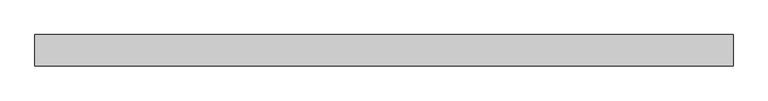
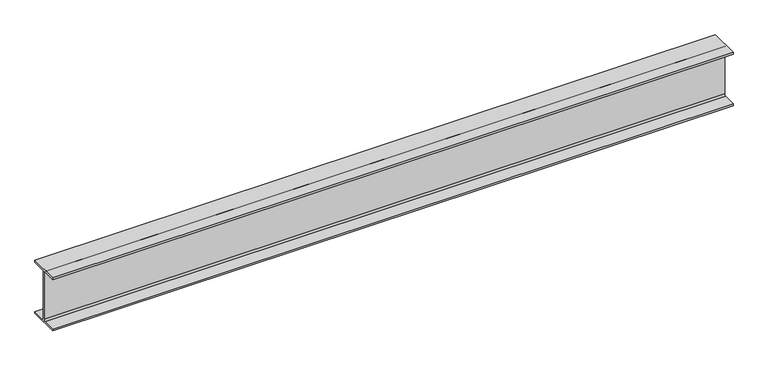
"""IFC4 building model written with IfcOpenShell, lengths in millimetres: beam geometry, Old_Steel Beam_H-KSD3502 : H_SB_ASB_H-200×200x8x12."""

import ifcopenshell
import ifcopenshell.guid

model = None  # the IFC model being written
_history = None  # IfcOwnerHistory: only IFC2X3 demands one
_inside = {}  # id of a spatial element -> (the spatial element, [elements in it])
_under = {}  # id of a project, library or spatial element -> (it, [spatial elements below it])
_declared = {}  # id of a project -> (the project, [libraries it declares])
_typed = {}  # id of a type object -> (the type object, [elements of that type])
_made_of = {}  # id of a material, layer set ... -> (it, [elements and type objects made of it])


def new_model(schema):
    """Start an empty IFC model of exactly this schema.

    Asked for "IFC4X3", IfcOpenShell would pick the latest addendum, in which some entities
    have other attributes; the version numbers below select the first issue.
    IFC2X3 requires an IfcOwnerHistory on every rooted entity: one is made here for all.
    """
    global model, _history
    if schema == "IFC4X3":
        model = ifcopenshell.file(schema_version=(4, 3, 0, 0))
    else:
        model = ifcopenshell.file(schema=schema)
    _inside.clear()
    _under.clear()
    _declared.clear()
    _typed.clear()
    _made_of.clear()
    _history = None
    if model.schema == "IFC2X3":
        org = make("IfcOrganization", Name="unknown")
        user = make(
            "IfcPersonAndOrganization",
            ThePerson=make("IfcPerson", FamilyName="unknown"),
            TheOrganization=org,
        )
        app = make(
            "IfcApplication",
            ApplicationDeveloper=org,
            Version="unknown",
            ApplicationFullName="unknown",
            ApplicationIdentifier="unknown",
        )
        _history = make(
            "IfcOwnerHistory",
            OwningUser=user,
            OwningApplication=app,
            ChangeAction="ADDED",
            CreationDate=0,
        )
    return model


def make(cls, **values):
    """One entity of the class cls with the attributes given. An attribute that is None is left unset."""
    return model.create_entity(
        cls, **{name: value for name, value in values.items() if value is not None}
    )


def rooted(cls, **values):
    """An entity with a GlobalId (a new one), such as an element, a storey or a relation."""
    return make(cls, GlobalId=ifcopenshell.guid.new(), OwnerHistory=_history, **values)


def si_unit(unit_type, name, prefix=None):
    """IfcSIUnit, for example si_unit("LENGTHUNIT", "METRE", prefix="MILLI")."""
    return make("IfcSIUnit", UnitType=unit_type, Prefix=prefix, Name=name)


def assignment(units):
    """IfcUnitAssignment: the units of a project."""
    return None if units is None else make("IfcUnitAssignment", Units=units)


def point(xyz):
    """IfcCartesianPoint."""
    return None if xyz is None else make("IfcCartesianPoint", Coordinates=xyz)


def direction(xyz):
    """IfcDirection."""
    return None if xyz is None else make("IfcDirection", DirectionRatios=xyz)


def frame(location, z_axis=None, x_axis=None):
    """IfcAxis2Placement3D, a coordinate frame: its origin and axes. An axis left out is left unset."""
    return make(
        "IfcAxis2Placement3D",
        Location=point(location),
        Axis=direction(z_axis),
        RefDirection=direction(x_axis),
    )


def frame_2d(location, x_axis=None):
    """IfcAxis2Placement2D, a coordinate frame in the plane: its origin and x axis."""
    return make(
        "IfcAxis2Placement2D", Location=point(location), RefDirection=direction(x_axis)
    )


def origin():
    """The frame at (0, 0, 0) with its axes left unset."""
    return frame((0.0, 0.0, 0.0))


def place(relative_to, where):
    """IfcLocalPlacement: puts the frame where relative to a parent placement (None: the world)."""
    return make(
        "IfcLocalPlacement", PlacementRelTo=relative_to, RelativePlacement=where
    )


def context(
    kind, dimensions, precision=None, world=None, true_north=None, identifier=None
):
    """IfcGeometricRepresentationContext, for example the 3D "Model" context."""
    return make(
        "IfcGeometricRepresentationContext",
        ContextIdentifier=identifier,
        ContextType=kind,
        CoordinateSpaceDimension=dimensions,
        Precision=precision,
        WorldCoordinateSystem=world,
        TrueNorth=true_north,
    )


def project(units=None, contexts=None):
    """IfcProject with its units and contexts."""
    return rooted(
        "IfcProject",
        Name="project",
        RepresentationContexts=contexts,
        UnitsInContext=assignment(units),
    )


def spatial(cls, under=None, at=None, **own):
    """A site, building, storey or space (cls), placed at a placement, below another one or the project."""
    s = rooted(cls, ObjectPlacement=at, **own)
    if under is not None:
        _under.setdefault(under.id(), (under, []))[1].append(s)
    return s


def polyline(points):
    """IfcPolyline through the points."""
    return make("IfcPolyline", Points=[point(p) for p in points])


def circle_curve(where, radius):
    """IfcCircle in the frame where."""
    return make("IfcCircle", Position=where, Radius=radius)


def trimmed(basis, trim1, trim2, sense, master):
    """IfcTrimmedCurve: the piece of a basis curve between two trims."""
    return make(
        "IfcTrimmedCurve",
        BasisCurve=basis,
        Trim1=trim1,
        Trim2=trim2,
        SenseAgreement=sense,
        MasterRepresentation=master,
    )


def segment(curve, same_sense, transition):
    """IfcCompositeCurveSegment."""
    return make(
        "IfcCompositeCurveSegment",
        Transition=transition,
        SameSense=same_sense,
        ParentCurve=curve,
    )


def composite_curve(segments, self_intersect=None):
    """IfcCompositeCurve: segments joined end to end."""
    return make("IfcCompositeCurve", Segments=segments, SelfIntersect=self_intersect)


def outline(outer, holes=None, kind="AREA"):
    """IfcArbitraryClosedProfileDef: a profile drawn as a closed curve; with holes, ...WithVoids."""
    if holes is None:
        return make("IfcArbitraryClosedProfileDef", ProfileType=kind, OuterCurve=outer)
    return make(
        "IfcArbitraryProfileDefWithVoids",
        ProfileType=kind,
        OuterCurve=outer,
        InnerCurves=holes,
    )


def extrude(swept, where, along, depth):
    """IfcExtrudedAreaSolid: the profile swept, set in the frame where, extruded along a direction by depth."""
    return make(
        "IfcExtrudedAreaSolid",
        SweptArea=swept,
        Position=where,
        ExtrudedDirection=direction(along),
        Depth=depth,
    )


def shape(context_of_items, identifier, shape_type, items):
    """IfcShapeRepresentation: the items that make up one representation, for example the "Body"."""
    return make(
        "IfcShapeRepresentation",
        ContextOfItems=context_of_items,
        RepresentationIdentifier=identifier,
        RepresentationType=shape_type,
        Items=items,
    )


def source(mapping_origin, context_of_items, identifier, shape_type, items):
    """IfcRepresentationMap: a shape defined once, which mapped items show again and again."""
    return make(
        "IfcRepresentationMap",
        MappingOrigin=mapping_origin,
        MappedRepresentation=shape(context_of_items, identifier, shape_type, items),
    )


def transform(
    local_origin,
    x_axis=None,
    y_axis=None,
    z_axis=None,
    scale=None,
    scale2=None,
    scale3=None,
    uniform=True,
):
    """IfcCartesianTransformationOperator3D, or its non-uniform kind. x_axis, y_axis, z_axis: its Axis1, 2, 3."""
    if uniform:
        return make(
            "IfcCartesianTransformationOperator3D",
            Axis1=direction(x_axis),
            Axis2=direction(y_axis),
            LocalOrigin=point(local_origin),
            Scale=scale,
            Axis3=direction(z_axis),
        )
    return make(
        "IfcCartesianTransformationOperator3DnonUniform",
        Axis1=direction(x_axis),
        Axis2=direction(y_axis),
        LocalOrigin=point(local_origin),
        Scale=scale,
        Axis3=direction(z_axis),
        Scale2=scale2,
        Scale3=scale3,
    )


def mapped(mapping_source, mapping_target):
    """IfcMappedItem: shows the shape of a source again, moved by a transform."""
    return make(
        "IfcMappedItem", MappingSource=mapping_source, MappingTarget=mapping_target
    )


def made_of(thing, what):
    """Note that an element or type object is made of a material, layer set ...; save() writes the relation."""
    if what is not None:
        _made_of.setdefault(what.id(), (what, []))[1].append(thing)
    return thing


def element(
    cls,
    number,
    at=None,
    inside=None,
    cuts=None,
    type_object=None,
    material=None,
    context=None,
    identifier="Body",
    shape_type=None,
    held_by="IfcProductDefinitionShape",
    body=None,
    shapes=None,
    **own,
):
    """One element of the class cls, such as IfcWall. Its Tag is "e" and its number.

    at: its placement. inside: the storey or other place that contains it. cuts: it is an
    opening in that element (IfcRelVoidsElement). A single representation is given by context,
    identifier, shape_type and body (its items); several are given by shapes. held_by: the class
    of the entity that holds the representations. save() writes the other relations.
    """
    e = rooted(cls, Tag="e%d" % number, ObjectPlacement=at, **own)
    if body is not None:
        shapes = [shape(context, identifier, shape_type, body)]
    if shapes is not None:
        e.Representation = make(held_by, Representations=shapes)
    if inside is not None:
        _inside.setdefault(inside.id(), (inside, []))[1].append(e)
    if cuts is not None:
        rooted(
            "IfcRelVoidsElement", RelatingBuildingElement=cuts, RelatedOpeningElement=e
        )
    if type_object is not None:
        _typed.setdefault(type_object.id(), (type_object, []))[1].append(e)
    return made_of(e, material)


def aggregate(whole, parts):
    """IfcRelAggregates: a whole, such as a stair, and the parts it consists of."""
    return rooted("IfcRelAggregates", RelatingObject=whole, RelatedObjects=parts)


def save(model, path):
    """Write the relations noted so far, then the file.

    IfcRelAggregates (storeys below a building ...), IfcRelContainedInSpatialStructure (elements
    in a storey), IfcRelDefinesByType, IfcRelAssociatesMaterial and IfcRelDeclares: one each for
    every whole, place, type object, material and project.
    """
    for whole, parts in _under.values():
        aggregate(whole, parts)
    for where, things in _inside.values():
        rooted(
            "IfcRelContainedInSpatialStructure",
            RelatedElements=things,
            RelatingStructure=where,
        )
    for kind, things in _typed.values():
        rooted("IfcRelDefinesByType", RelatedObjects=things, RelatingType=kind)
    for what, things in _made_of.values():
        rooted("IfcRelAssociatesMaterial", RelatedObjects=things, RelatingMaterial=what)
    for by, libraries in _declared.values():
        rooted("IfcRelDeclares", RelatingContext=by, RelatedDefinitions=libraries)
    model.write(path)


def beam_556eb451(model_context):
    return source(origin(), model_context, "Body", "SweptSolid", [
        extrude(outline(composite_curve([segment(polyline([(-82.5, -141.5), (-11.9, -141.5)]), True, "CONTINUOUS"), segment(trimmed(circle_curve(frame_2d((-11.9, -132.6)), 8.9), [point((-11.9, -141.5))], [point((-3.0, -132.6))], True, "CARTESIAN"), True, "CONTINUOUS"), segment(polyline([(-3.0, -132.6), (-3.0, 132.6)]), True, "CONTINUOUS"), segment(trimmed(circle_curve(frame_2d((-11.9, 132.6)), 8.9), [point((-3.0, 132.6))], [point((-11.9, 141.5))], True, "CARTESIAN"), True, "CONTINUOUS"), segment(polyline([(-11.9, 141.5), (-82.5, 141.5), (-82.5, 151.7), (82.5, 151.7), (82.5, 141.5), (11.9, 141.5)]), True, "CONTINUOUS"), segment(trimmed(circle_curve(frame_2d((11.9, 132.6)), 8.9), [point((11.9, 141.5))], [point((3.0, 132.6))], True, "CARTESIAN"), True, "CONTINUOUS"), segment(polyline([(3.0, 132.6), (3.0, -132.6)]), True, "CONTINUOUS"), segment(trimmed(circle_curve(frame_2d((11.9, -132.6)), 8.9), [point((3.0, -132.6))], [point((11.9, -141.5))], True, "CARTESIAN"), True, "CONTINUOUS"), segment(polyline([(11.9, -141.5), (82.5, -141.5), (82.5, -151.7), (-82.5, -151.7), (-82.5, -141.5)]), True, "CONTINUOUS")], self_intersect=False)), frame((-1848.779151, 0.0, 0.0), z_axis=(1.0, 0.0, 0.0), x_axis=(0.0, 1.0, 0.0)), (0.0, 0.0, 1.0), 3672.4688696),
    ])


if __name__ == "__main__":
    model = new_model("IFC4")
    model_context = context("Model", 3, world=origin())
    ifc_project = project(units=[si_unit("LENGTHUNIT", "METRE", prefix="MILLI")], contexts=[model_context])
    site = spatial("IfcSite", under=ifc_project)
    building = spatial("IfcBuilding", under=site)
    placement = place(None, origin())
    beam_shape = beam_556eb451(model_context)
    element("IfcBeam", 1, ObjectType="Old_Steel Beam_H-KSD3502 : H_SB_ASB_H-200×200x8x12", at=placement, inside=building, context=model_context, shape_type="MappedRepresentation", body=[
        mapped(beam_shape, transform((0.0, 0.0, 0.0), x_axis=(1.0, 0.0, 0.0), y_axis=(0.0, 1.0, 0.0), z_axis=(0.0, 0.0, 1.0))),
    ])
    save(model, "model.ifc")

# Revit data of these elements
# Type "Old_Steel Beam_H-KSD3502 : H_SB_ASB_H-200×200x8x12"
#   Width = 20.0 cm
#   Web Thickness = 0.8 cm
#   Web Fillet = 1.3 cm
#   Warping Constant = 141376.0 cm⁶
#   Torsional Moment of Inertia = 26.2485 cm⁴
#   Torsional Modulus = 1.0 cm³
#   Section Area = 63.53 cm²
#   Plastic Modulus weak axis = 244.0 cm³
#   Plastic Modulus strong axis = 525.0 cm³
#   Perimeter = 1.16 m²/m
#   Nominal Weight = 49.90 kgf/m
#   Moment of Inertia weak axis = 1600.00 cm⁴
#   Moment of Inertia strong axis = 4720.00 cm⁴
#   Height = 20.0 cm
#   Flange Thickness = 1.2 cm
#   Elastic Modulus weak axis = 160.0 cm³
#   Elastic Modulus strong axis = 472.0 cm³
#   Centroid Vertical = 10.0 cm
#   Centroid Horizontal = 10.0 cm
#   Length [instance default] = 1.5240 m
#   Structural Material [instance default] = Steel, 45-345
#   Assembly Code = ""
# Element 1 (IfcBeam, "Old_Steel Beam_H-KSD3502 : H_SB_ASB_H-200×200x8x12")
#   Structural Material = none
# Materials
#   "Steel, 45-345": class "Metal", colour RGB 189 187 185, transparency 0, Description = "Steel 345 MPa", Cost = 0
